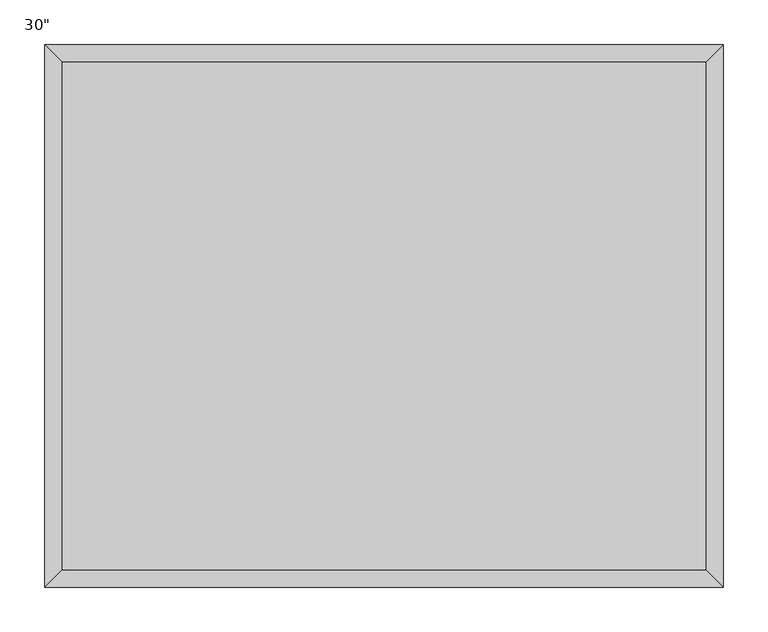
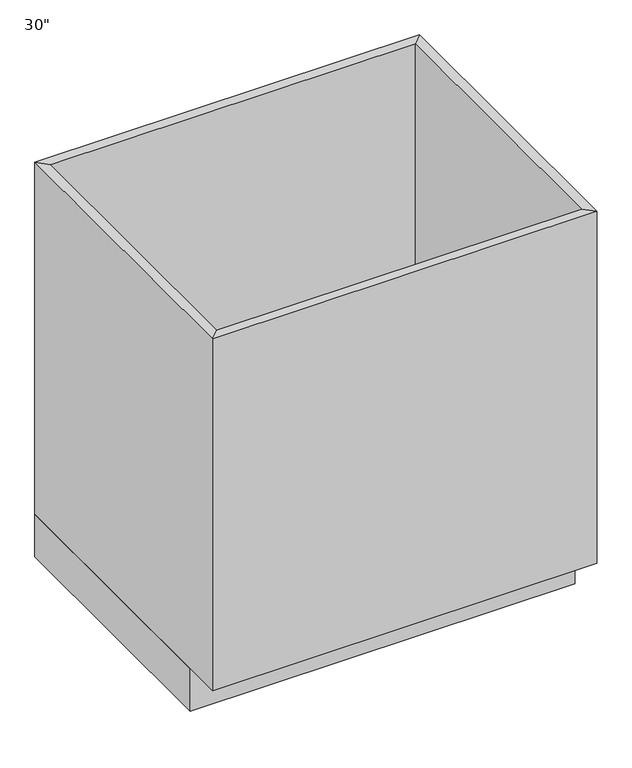
"""IFC4 building model written with IfcOpenShell, lengths in millimetres: furniture geometry."""

from ifc_helpers import new_model, si_unit, frame, origin, origin_with_axes, place, context, project, spatial, polyline, outline, extrude, faceted_brep, source, transform, mapped, element, save


def furniture_6ba5c079(model_context):
    return source(origin(), model_context, "Body", "SolidModel", [
        extrude(outline(polyline([(380.6877049, -19.05), (380.6877049, -590.55), (-343.2122951, -590.55), (-343.2122951, -19.05), (380.6877049, -19.05)])), frame((0.0, 0.0, 88.9), z_axis=(0.0, 0.0, 1.0), x_axis=(1.0, 0.0, 0.0)), (0.0, 0.0, 1.0), 19.05),
        faceted_brep([(380.6877049, -590.55, 825.5), (380.6877049, -590.55, 88.9), (-343.2122951, -590.55, 88.9), (-343.2122951, -590.55, 825.5), (399.7377049, -609.6, 825.5), (-362.2622951, -609.6, 825.5), (399.7377049, -609.6, 88.9), (-362.2622951, -609.6, 88.9), (-343.2122951, -19.05, 88.9), (-343.2122951, -19.05, 825.5), (-362.2622951, 0.0, 825.5), (-362.2622951, 0.0, 88.9), (380.6877049, -19.05, 88.9), (380.6877049, -19.05, 825.5), (399.7377049, 0.0, 825.5), (399.7377049, 0.0, 88.9)], [[[0, 1, 2, 3]], [[4, 0, 3, 5]], [[6, 4, 5, 7]], [[1, 6, 7, 2]], [[3, 2, 8, 9]], [[5, 3, 9, 10]], [[7, 5, 10, 11]], [[2, 7, 11, 8]], [[9, 8, 12, 13]], [[10, 9, 13, 14]], [[11, 10, 14, 15]], [[8, 11, 15, 12]], [[13, 12, 1, 0]], [[14, 13, 0, 4]], [[15, 14, 4, 6]], [[12, 15, 6, 1]]]),
        extrude(outline(polyline([(399.7377049, 0.0), (399.7377049, -533.4), (-362.2622951, -533.4), (-362.2622951, 0.0), (399.7377049, 0.0)])), origin_with_axes(), (0.0, 0.0, 1.0), 88.9),
    ])


if __name__ == "__main__":
    model = new_model("IFC4")
    model_context = context("Model", 3, world=origin())
    ifc_project = project(units=[si_unit("LENGTHUNIT", "METRE", prefix="MILLI")], contexts=[model_context])
    site = spatial("IfcSite", under=ifc_project)
    building = spatial("IfcBuilding", under=site)
    placement = place(None, origin())
    furniture_shape = furniture_6ba5c079(model_context)
    element("IfcFurniture", 1, ObjectType="Base Cabinet-Double Door & 1 Drawer : 30\"", at=placement, inside=building, context=model_context, shape_type="MappedRepresentation", body=[
        mapped(furniture_shape, transform((0.0, 0.0, 0.0), x_axis=(1.0, 0.0, 0.0), y_axis=(0.0, 1.0, 0.0), z_axis=(0.0, 0.0, 1.0))),
    ])
    save(model, "model.ifc")

# Revit data of these elements
# Type "Base Cabinet-Double Door & 1 Drawer : 30\""
#   Finish = "Cabinetry"
#   Finish = "Cabinet"
#   Depth = 2' - 0"
#   Height = 2' - 8 1/2"
#   Toe Depth = 0' - 3"
#   Toe Height = 0' - 3 1/2"
#   Width = 2' - 6"
#   Cabinet Material = none
# Element 1 (IfcFurniture, "Base Cabinet-Double Door & 1 Drawer : 30\"")
#   Materials on its faces: "CASEWORK"
# Materials
#   "CASEWORK": class "Generic", colour RGB 181 181 181, transparency 0, Cost = 0
